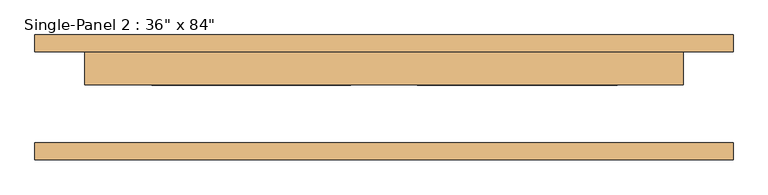
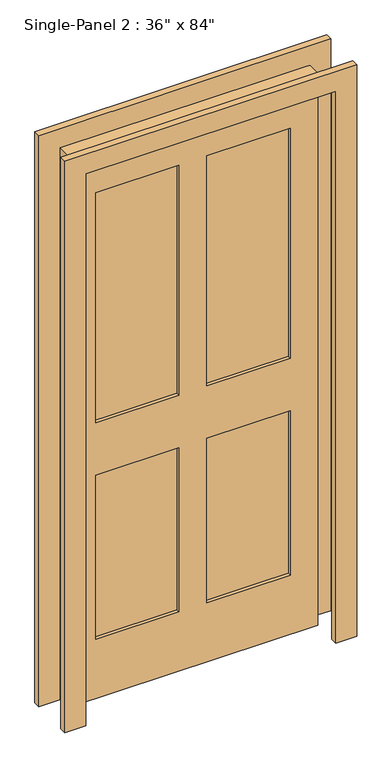
"""IFC4 building model written with IfcOpenShell, lengths in millimetres: door geometry."""

from ifc_helpers import new_model, si_unit, frame, origin, place, context, project, spatial, polyline, outline, extrude, source, transform, mapped, element, save


def door_0975cc44(model_context):
    return source(origin(), model_context, "Body", "SweptSolid", [
        extrude(outline(polyline([(-50.9240165, 31.75), (-355.0511799, 31.75), (-355.0511799, 57.15), (-50.9240165, 57.15), (-50.9240165, 31.75)])), frame((0.0, 0.0, 1068.1906173), z_axis=(0.0, 0.0, 1.0), x_axis=(1.0, 0.0, 0.0)), (0.0, 0.0, 1.0), 889.2046757),
        extrude(outline(polyline([(356.1488201, 31.75), (50.6759835, 31.75), (50.6759835, 57.15), (356.1488201, 57.15), (356.1488201, 31.75)])), frame((0.0, 0.0, 1068.1906173), z_axis=(0.0, 0.0, 1.0), x_axis=(1.0, 0.0, 0.0)), (0.0, 0.0, 1.0), 889.2046757),
        extrude(outline(polyline([(-50.9240165, 31.75), (-355.0511799, 31.75), (-355.0511799, 57.15), (-50.9240165, 57.15), (-50.9240165, 31.75)])), frame((0.0, 0.0, 230.195293), z_axis=(0.0, 0.0, 1.0), x_axis=(1.0, 0.0, 0.0)), (0.0, 0.0, 1.0), 635.0),
        extrude(outline(polyline([(356.1488201, 31.75), (50.6759835, 31.75), (50.6759835, 57.15), (356.1488201, 57.15), (356.1488201, 31.75)])), frame((0.0, 0.0, 230.195293), z_axis=(0.0, 0.0, 1.0), x_axis=(1.0, 0.0, 0.0)), (0.0, 0.0, 1.0), 634.7953243),
        extrude(outline(polyline([(2209.8, -533.4), (1.3906173, -533.4), (1.3906173, -457.3240165), (2134.9906173, -457.3240165), (2134.9906173, 457.0759835), (1.3906173, 457.0759835), (0.0, 533.4), (2209.8, 533.4), (2209.8, -533.4)])), frame((0.0, 69.85, 0.0), z_axis=(0.0, 1.0, 0.0), x_axis=(0.0, 0.0, 1.0)), (0.0, 0.0, 1.0), 25.4),
        extrude(outline(polyline([(2209.8, 533.4), (2209.8, -533.4), (1.3906173, -533.4), (1.3906173, -457.3240165), (2134.9906173, -457.3240165), (2134.9906173, 457.0759835), (1.3906173, 457.0759835), (0.0, 533.4), (2209.8, 533.4)])), frame((0.0, -95.25, 0.0), z_axis=(0.0, 1.0, 0.0), x_axis=(0.0, 0.0, 1.0)), (0.0, 0.0, 1.0), 25.4),
        extrude(outline(polyline([(2134.9906173, 457.0759835), (2134.9906173, -457.3240165), (1.3906173, -457.3240165), (1.3906173, 457.0759835), (2134.9906173, 457.0759835)]), holes=[polyline([(1957.395293, -50.9240165), (1068.1906173, -50.9240165), (1068.1906173, -355.0511799), (1957.395293, -355.0511799), (1957.395293, -50.9240165)]), polyline([(1957.395293, 356.1488201), (1068.1906173, 356.1488201), (1068.1906173, 50.6759835), (1957.395293, 50.6759835), (1957.395293, 356.1488201)]), polyline([(865.195293, -50.9240165), (230.195293, -50.9240165), (230.195293, -355.0511799), (865.195293, -355.0511799), (865.195293, -50.9240165)]), polyline([(864.9906173, 356.1488201), (230.195293, 356.1488201), (230.195293, 50.6759835), (864.9906173, 50.6759835), (864.9906173, 356.1488201)])]), frame((0.0, 19.05, 0.0), z_axis=(0.0, 1.0, 0.0), x_axis=(0.0, 0.0, 1.0)), (0.0, 0.0, 1.0), 50.8),
    ])


if __name__ == "__main__":
    model = new_model("IFC4")
    model_context = context("Model", 3, world=origin())
    ifc_project = project(units=[si_unit("LENGTHUNIT", "METRE", prefix="MILLI")], contexts=[model_context])
    site = spatial("IfcSite", under=ifc_project)
    building = spatial("IfcBuilding", under=site)
    placement = place(None, origin())
    door_shape = door_0975cc44(model_context)
    element("IfcDoor", 1, ObjectType="Single-Panel 2 : 36\" x 84\"", at=placement, inside=building, context=model_context, shape_type="MappedRepresentation", body=[
        mapped(door_shape, transform((0.0, 0.0, 0.0), x_axis=(1.0, 0.0, 0.0), y_axis=(0.0, 1.0, 0.0), z_axis=(0.0, 0.0, 1.0))),
    ])
    save(model, "model.ifc")

# Revit data of these elements
# Type "Single-Panel 2 : 36\" x 84\""
#   Type Mark = "6"
#   Assembly Code = "C1020"
#   Thickness = 0' - 2"
#   Height = 7' - 0"
#   Rail Width - Base = 0' - 9"
#   Rail Width - Center = 0' - 8"
#   Rail Width - Top = 0' - 7"
#   Stile Width = 0' - 4"
#   Trim Projection Ext = 0' - 1"
#   Trim Projection Int = 0' - 1"
#   Trim Width = 0' - 3"
#   Width = 3' - 0"
#   Function = 0
#   Door Material = Door - Panel
#   Frame Material = Door - Frame
#   Wall Closure = (empty or 0)
# Element 1 (IfcDoor, "Single-Panel 2 : 36\" x 84\"")
#   Materials on its faces: "Door - Panel", "Door - Frame"
# Materials
#   "Door - Panel": class "Wood", colour RGB 149 143 132, transparency 0, Comments = "Rendering appearance not upgraded Rendering appearance not upgraded "
#   "Door - Frame": class "Unassigned", colour RGB 118 70 51, transparency 0, Comments = "Rendering appearance not upgraded Rendering appearance not upgraded "
